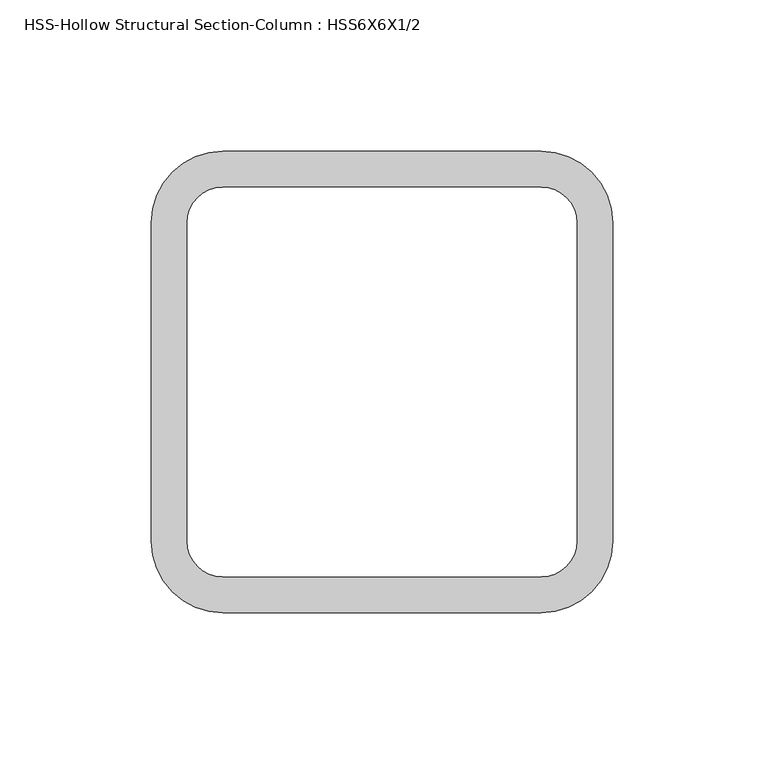
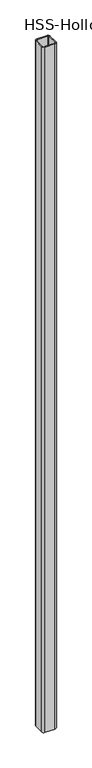
"""IFC4 building model written with IfcOpenShell, lengths in millimetres: column geometry, HSS-Hollow Structural Section-Column : HSS6X6X1/2."""

from ifc_helpers import new_model, si_unit, point, frame, frame_2d, origin, place, context, project, spatial, polyline, circle_curve, trimmed, segment, composite_curve, outline, extrude, source, transform, mapped, element, save


def hss_hollow_structural_section_column_hss6x6x1_2_d5a0f1ec(model_context):
    return source(origin(), model_context, "Body", "SweptSolid", [
        extrude(outline(composite_curve([segment(trimmed(circle_curve(frame_2d((52.578, 52.578)), 23.622), [point((52.578, 76.2))], [point((76.2, 52.578))], False, "CARTESIAN"), True, "CONTINUOUS"), segment(polyline([(76.2, 52.578), (76.2, -52.578)]), True, "CONTINUOUS"), segment(trimmed(circle_curve(frame_2d((52.578, -52.578)), 23.622), [point((76.2, -52.578))], [point((52.578, -76.2))], False, "CARTESIAN"), True, "CONTINUOUS"), segment(polyline([(52.578, -76.2), (-52.578, -76.2)]), True, "CONTINUOUS"), segment(trimmed(circle_curve(frame_2d((-52.578, -52.578)), 23.622), [point((-52.578, -76.2))], [point((-76.2, -52.578))], False, "CARTESIAN"), True, "CONTINUOUS"), segment(polyline([(-76.2, -52.578), (-76.2, 52.578)]), True, "CONTINUOUS"), segment(trimmed(circle_curve(frame_2d((-52.578, 52.578)), 23.622), [point((-76.2, 52.578))], [point((-52.578, 76.2))], False, "CARTESIAN"), True, "CONTINUOUS"), segment(polyline([(-52.578, 76.2), (52.578, 76.2)]), True, "CONTINUOUS")], self_intersect=False), holes=[composite_curve([segment(polyline([(52.578, 64.389), (-52.578, 64.389)]), True, "CONTINUOUS"), segment(trimmed(circle_curve(frame_2d((-52.578, 52.578)), 11.811), [point((-52.578, 64.389))], [point((-64.389, 52.578))], True, "CARTESIAN"), True, "CONTINUOUS"), segment(polyline([(-64.389, 52.578), (-64.389, -52.578)]), True, "CONTINUOUS"), segment(trimmed(circle_curve(frame_2d((-52.578, -52.578)), 11.811), [point((-64.389, -52.578))], [point((-52.578, -64.389))], True, "CARTESIAN"), True, "CONTINUOUS"), segment(polyline([(-52.578, -64.389), (52.578, -64.389)]), True, "CONTINUOUS"), segment(trimmed(circle_curve(frame_2d((52.578, -52.578)), 11.811), [point((52.578, -64.389))], [point((64.389, -52.578))], True, "CARTESIAN"), True, "CONTINUOUS"), segment(polyline([(64.389, -52.578), (64.389, 52.578)]), True, "CONTINUOUS"), segment(trimmed(circle_curve(frame_2d((52.578, 52.578)), 11.811), [point((64.389, 52.578))], [point((52.578, 64.389))], True, "CARTESIAN"), True, "CONTINUOUS")], self_intersect=False)]), frame((0.0, 0.0, 4267.2), z_axis=(0.0, 0.0, 1.0), x_axis=(1.0, 0.0, 0.0)), (0.0, 0.0, 1.0), 7721.6),
    ])


if __name__ == "__main__":
    model = new_model("IFC4")
    model_context = context("Model", 3, world=origin())
    ifc_project = project(units=[si_unit("LENGTHUNIT", "METRE", prefix="MILLI")], contexts=[model_context])
    site = spatial("IfcSite", under=ifc_project)
    building = spatial("IfcBuilding", under=site)
    placement = place(None, origin())
    hss_hollow_structural_section_column_hss6x6x1_2_shape = hss_hollow_structural_section_column_hss6x6x1_2_d5a0f1ec(model_context)
    element("IfcColumn", 1, ObjectType="HSS-Hollow Structural Section-Column : HSS6X6X1/2", at=placement, inside=building, context=model_context, shape_type="MappedRepresentation", body=[
        mapped(hss_hollow_structural_section_column_hss6x6x1_2_shape, transform((0.0, 0.0, 0.0), x_axis=(1.0, 0.0, 0.0), y_axis=(0.0, 1.0, 0.0), z_axis=(0.0, 0.0, 1.0))),
    ])
    save(model, "model.ifc")

# Revit data of these elements
# Type "HSS-Hollow Structural Section-Column : HSS6X6X1/2"
#   Assembly Code = "B10"
#   Shape = "Square"
#   W = 35.1
#   Ht = 0' - 6"
#   b = 0' - 6"
#   kr = 0' - 0.93"
#   t = 0' - 0.465"
#   A = 0.0676389 SF
#   Structural Material [instance default] = Steel ASTM A500, Grade B, Rectangular and Square
# Element 1 (IfcColumn, "HSS-Hollow Structural Section-Column : HSS6X6X1/2")
#   Materials on its faces: "Steel ASTM A500, Grade B, Rectangular and Square"
# Materials
#   "Steel ASTM A500, Grade B, Rectangular and Square": class "Metal", colour RGB 199 199 199, transparency 0, Description = "Carbon steel", Cost = 0
